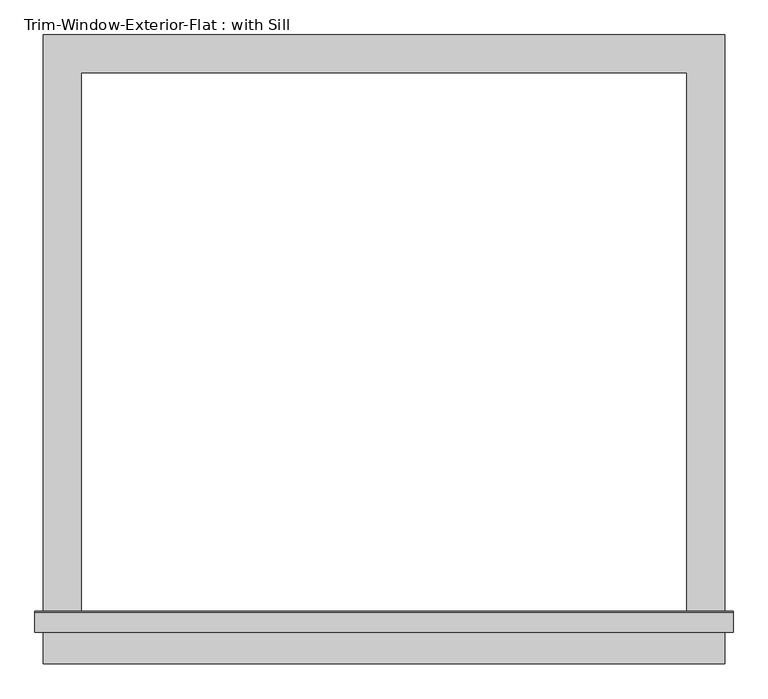
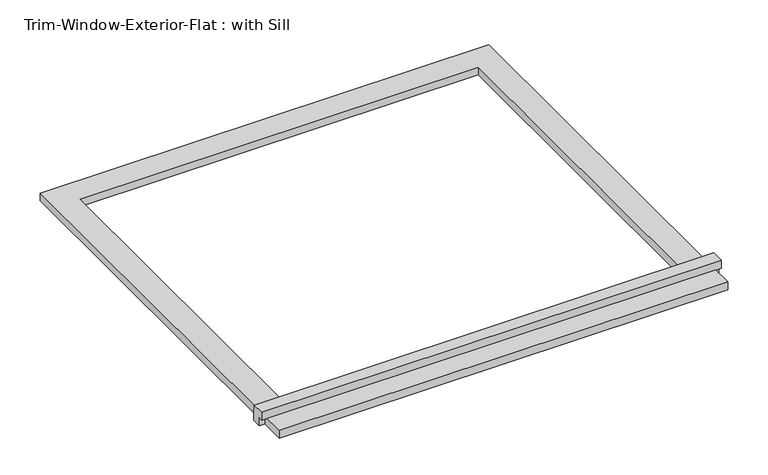
"""IFC4 building model written with IfcOpenShell, lengths in millimetres: proxy geometry, Trim-Window-Exterior-Flat : with Sill."""

import ifcopenshell
import ifcopenshell.guid

model = None  # the IFC model being written
_history = None  # IfcOwnerHistory: only IFC2X3 demands one
_inside = {}  # id of a spatial element -> (the spatial element, [elements in it])
_under = {}  # id of a project, library or spatial element -> (it, [spatial elements below it])
_declared = {}  # id of a project -> (the project, [libraries it declares])
_typed = {}  # id of a type object -> (the type object, [elements of that type])
_made_of = {}  # id of a material, layer set ... -> (it, [elements and type objects made of it])


def new_model(schema):
    """Start an empty IFC model of exactly this schema.

    Asked for "IFC4X3", IfcOpenShell would pick the latest addendum, in which some entities
    have other attributes; the version numbers below select the first issue.
    IFC2X3 requires an IfcOwnerHistory on every rooted entity: one is made here for all.
    """
    global model, _history
    if schema == "IFC4X3":
        model = ifcopenshell.file(schema_version=(4, 3, 0, 0))
    else:
        model = ifcopenshell.file(schema=schema)
    _inside.clear()
    _under.clear()
    _declared.clear()
    _typed.clear()
    _made_of.clear()
    _history = None
    if model.schema == "IFC2X3":
        org = make("IfcOrganization", Name="unknown")
        user = make(
            "IfcPersonAndOrganization",
            ThePerson=make("IfcPerson", FamilyName="unknown"),
            TheOrganization=org,
        )
        app = make(
            "IfcApplication",
            ApplicationDeveloper=org,
            Version="unknown",
            ApplicationFullName="unknown",
            ApplicationIdentifier="unknown",
        )
        _history = make(
            "IfcOwnerHistory",
            OwningUser=user,
            OwningApplication=app,
            ChangeAction="ADDED",
            CreationDate=0,
        )
    return model


def make(cls, **values):
    """One entity of the class cls with the attributes given. An attribute that is None is left unset."""
    return model.create_entity(
        cls, **{name: value for name, value in values.items() if value is not None}
    )


def rooted(cls, **values):
    """An entity with a GlobalId (a new one), such as an element, a storey or a relation."""
    return make(cls, GlobalId=ifcopenshell.guid.new(), OwnerHistory=_history, **values)


def si_unit(unit_type, name, prefix=None):
    """IfcSIUnit, for example si_unit("LENGTHUNIT", "METRE", prefix="MILLI")."""
    return make("IfcSIUnit", UnitType=unit_type, Prefix=prefix, Name=name)


def assignment(units):
    """IfcUnitAssignment: the units of a project."""
    return None if units is None else make("IfcUnitAssignment", Units=units)


def point(xyz):
    """IfcCartesianPoint."""
    return None if xyz is None else make("IfcCartesianPoint", Coordinates=xyz)


def direction(xyz):
    """IfcDirection."""
    return None if xyz is None else make("IfcDirection", DirectionRatios=xyz)


def frame(location, z_axis=None, x_axis=None):
    """IfcAxis2Placement3D, a coordinate frame: its origin and axes. An axis left out is left unset."""
    return make(
        "IfcAxis2Placement3D",
        Location=point(location),
        Axis=direction(z_axis),
        RefDirection=direction(x_axis),
    )


def origin():
    """The frame at (0, 0, 0) with its axes left unset."""
    return frame((0.0, 0.0, 0.0))


def origin_with_axes():
    """The frame at (0, 0, 0) with the z axis (0, 0, 1) and the x axis (1, 0, 0) written out."""
    return frame((0.0, 0.0, 0.0), z_axis=(0.0, 0.0, 1.0), x_axis=(1.0, 0.0, 0.0))


def place(relative_to, where):
    """IfcLocalPlacement: puts the frame where relative to a parent placement (None: the world)."""
    return make(
        "IfcLocalPlacement", PlacementRelTo=relative_to, RelativePlacement=where
    )


def context(
    kind, dimensions, precision=None, world=None, true_north=None, identifier=None
):
    """IfcGeometricRepresentationContext, for example the 3D "Model" context."""
    return make(
        "IfcGeometricRepresentationContext",
        ContextIdentifier=identifier,
        ContextType=kind,
        CoordinateSpaceDimension=dimensions,
        Precision=precision,
        WorldCoordinateSystem=world,
        TrueNorth=true_north,
    )


def project(units=None, contexts=None):
    """IfcProject with its units and contexts."""
    return rooted(
        "IfcProject",
        Name="project",
        RepresentationContexts=contexts,
        UnitsInContext=assignment(units),
    )


def spatial(cls, under=None, at=None, **own):
    """A site, building, storey or space (cls), placed at a placement, below another one or the project."""
    s = rooted(cls, ObjectPlacement=at, **own)
    if under is not None:
        _under.setdefault(under.id(), (under, []))[1].append(s)
    return s


def polyline(points):
    """IfcPolyline through the points."""
    return make("IfcPolyline", Points=[point(p) for p in points])


def outline(outer, holes=None, kind="AREA"):
    """IfcArbitraryClosedProfileDef: a profile drawn as a closed curve; with holes, ...WithVoids."""
    if holes is None:
        return make("IfcArbitraryClosedProfileDef", ProfileType=kind, OuterCurve=outer)
    return make(
        "IfcArbitraryProfileDefWithVoids",
        ProfileType=kind,
        OuterCurve=outer,
        InnerCurves=holes,
    )


def extrude(swept, where, along, depth):
    """IfcExtrudedAreaSolid: the profile swept, set in the frame where, extruded along a direction by depth."""
    return make(
        "IfcExtrudedAreaSolid",
        SweptArea=swept,
        Position=where,
        ExtrudedDirection=direction(along),
        Depth=depth,
    )


def shape(context_of_items, identifier, shape_type, items):
    """IfcShapeRepresentation: the items that make up one representation, for example the "Body"."""
    return make(
        "IfcShapeRepresentation",
        ContextOfItems=context_of_items,
        RepresentationIdentifier=identifier,
        RepresentationType=shape_type,
        Items=items,
    )


def source(mapping_origin, context_of_items, identifier, shape_type, items):
    """IfcRepresentationMap: a shape defined once, which mapped items show again and again."""
    return make(
        "IfcRepresentationMap",
        MappingOrigin=mapping_origin,
        MappedRepresentation=shape(context_of_items, identifier, shape_type, items),
    )


def transform(
    local_origin,
    x_axis=None,
    y_axis=None,
    z_axis=None,
    scale=None,
    scale2=None,
    scale3=None,
    uniform=True,
):
    """IfcCartesianTransformationOperator3D, or its non-uniform kind. x_axis, y_axis, z_axis: its Axis1, 2, 3."""
    if uniform:
        return make(
            "IfcCartesianTransformationOperator3D",
            Axis1=direction(x_axis),
            Axis2=direction(y_axis),
            LocalOrigin=point(local_origin),
            Scale=scale,
            Axis3=direction(z_axis),
        )
    return make(
        "IfcCartesianTransformationOperator3DnonUniform",
        Axis1=direction(x_axis),
        Axis2=direction(y_axis),
        LocalOrigin=point(local_origin),
        Scale=scale,
        Axis3=direction(z_axis),
        Scale2=scale2,
        Scale3=scale3,
    )


def mapped(mapping_source, mapping_target):
    """IfcMappedItem: shows the shape of a source again, moved by a transform."""
    return make(
        "IfcMappedItem", MappingSource=mapping_source, MappingTarget=mapping_target
    )


def made_of(thing, what):
    """Note that an element or type object is made of a material, layer set ...; save() writes the relation."""
    if what is not None:
        _made_of.setdefault(what.id(), (what, []))[1].append(thing)
    return thing


def element(
    cls,
    number,
    at=None,
    inside=None,
    cuts=None,
    type_object=None,
    material=None,
    context=None,
    identifier="Body",
    shape_type=None,
    held_by="IfcProductDefinitionShape",
    body=None,
    shapes=None,
    **own,
):
    """One element of the class cls, such as IfcWall. Its Tag is "e" and its number.

    at: its placement. inside: the storey or other place that contains it. cuts: it is an
    opening in that element (IfcRelVoidsElement). A single representation is given by context,
    identifier, shape_type and body (its items); several are given by shapes. held_by: the class
    of the entity that holds the representations. save() writes the other relations.
    """
    e = rooted(cls, Tag="e%d" % number, ObjectPlacement=at, **own)
    if body is not None:
        shapes = [shape(context, identifier, shape_type, body)]
    if shapes is not None:
        e.Representation = make(held_by, Representations=shapes)
    if inside is not None:
        _inside.setdefault(inside.id(), (inside, []))[1].append(e)
    if cuts is not None:
        rooted(
            "IfcRelVoidsElement", RelatingBuildingElement=cuts, RelatedOpeningElement=e
        )
    if type_object is not None:
        _typed.setdefault(type_object.id(), (type_object, []))[1].append(e)
    return made_of(e, material)


def aggregate(whole, parts):
    """IfcRelAggregates: a whole, such as a stair, and the parts it consists of."""
    return rooted("IfcRelAggregates", RelatingObject=whole, RelatedObjects=parts)


def save(model, path):
    """Write the relations noted so far, then the file.

    IfcRelAggregates (storeys below a building ...), IfcRelContainedInSpatialStructure (elements
    in a storey), IfcRelDefinesByType, IfcRelAssociatesMaterial and IfcRelDeclares: one each for
    every whole, place, type object, material and project.
    """
    for whole, parts in _under.values():
        aggregate(whole, parts)
    for where, things in _inside.values():
        rooted(
            "IfcRelContainedInSpatialStructure",
            RelatedElements=things,
            RelatingStructure=where,
        )
    for kind, things in _typed.values():
        rooted("IfcRelDefinesByType", RelatedObjects=things, RelatingType=kind)
    for what, things in _made_of.values():
        rooted("IfcRelAssociatesMaterial", RelatedObjects=things, RelatingMaterial=what)
    for by, libraries in _declared.values():
        rooted("IfcRelDeclares", RelatingContext=by, RelatedDefinitions=libraries)
    model.write(path)


def trim_window_exterior_flat_with_sill_49d6f9d6(model_context):
    return source(origin(), model_context, "Body", "SweptSolid", [
        extrude(outline(polyline([(514.35, -834.9823709), (514.35, -892.1323709), (-514.35, -892.1323709), (-514.35, -834.9823709), (514.35, -834.9823709)])), origin_with_axes(), (0.0, 0.0, 1.0), 19.05),
        extrude(outline(polyline([(-844.55, 38.1), (-815.2580645, 38.1), (-812.8, 19.05), (-812.8, 0.0), (-834.9823709, 0.0), (-834.9823709, 19.05), (-844.55, 19.05), (-844.55, 38.1)])), frame((-527.05, 0.0, 0.0), z_axis=(1.0, 0.0, 0.0), x_axis=(0.0, 1.0, 0.0)), (0.0, 0.0, 1.0), 1054.1),
        extrude(outline(polyline([(-514.35, 57.15), (514.35, 57.15), (514.35, -812.8), (457.2, -812.8), (457.2, 0.0), (-457.2, 0.0), (-457.2, -812.8), (-514.35, -812.8), (-514.35, 57.15)])), origin_with_axes(), (0.0, 0.0, 1.0), 19.05),
    ])


if __name__ == "__main__":
    model = new_model("IFC4")
    model_context = context("Model", 3, world=origin())
    ifc_project = project(units=[si_unit("LENGTHUNIT", "METRE", prefix="MILLI")], contexts=[model_context])
    site = spatial("IfcSite", under=ifc_project)
    building = spatial("IfcBuilding", under=site)
    placement = place(None, origin())
    trim_window_exterior_flat_with_sill_shape = trim_window_exterior_flat_with_sill_49d6f9d6(model_context)
    element("IfcBuildingElementProxy", 1, Name="Trim-Window-Exterior-Flat : with Sill", ObjectType="Trim-Window-Exterior-Flat : with Sill", at=placement, inside=building, context=model_context, shape_type="MappedRepresentation", body=[
        mapped(trim_window_exterior_flat_with_sill_shape, transform((0.0, 0.0, 0.0), x_axis=(1.0, 0.0, 0.0), y_axis=(0.0, 1.0, 0.0), z_axis=(0.0, 0.0, 1.0))),
    ])
    save(model, "model.ifc")

# Revit data of these elements
# Type "Trim-Window-Exterior-Flat : with Sill"
#   Trim Width = 0' - 2 1/4"
#   Trim Thickness_Picture Frame = 0' - 1 1/4"
#   Trim Thickness_with Sill = 0' - 0 3/4"
#   Sill Thickness = 0' - 1 1/4"
#   Opening Width [instance default] = 2' - 0"
#   Opening Height [instance default] = 3' - 0"
#   Default Elevation = 4' - 0"
#   Sill = yes
#   Picture Frame = no
#   Trim Material [instance default] = none
# Element 1 (IfcBuildingElementProxy, "Trim-Window-Exterior-Flat : with Sill")
#   Opening Width = 3' - 0"
#   Opening Height = 2' - 8"
#   Trim Material = Clad - White
#   Materials on its faces: "Clad - White"
# Materials
#   "Clad - White": class "Wood", colour RGB 242 242 238, transparency 0, Cost = 0
